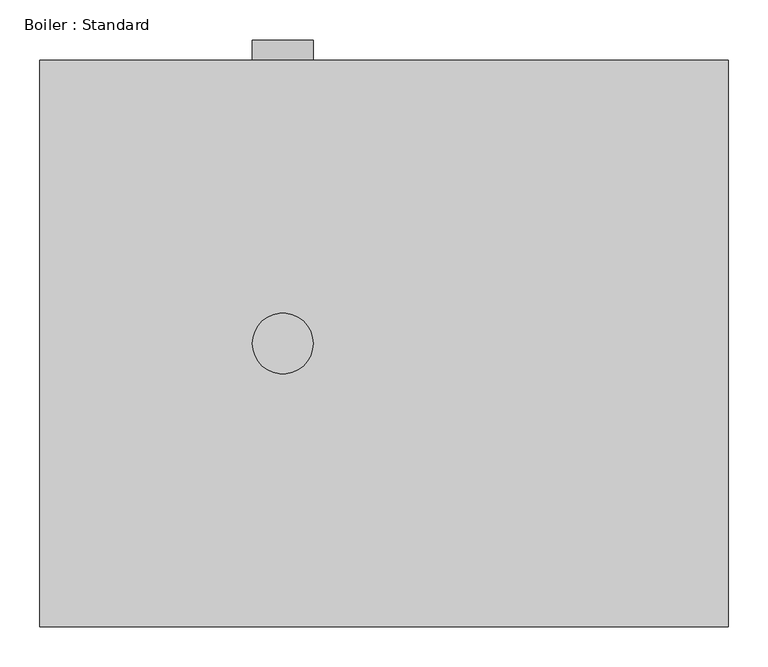
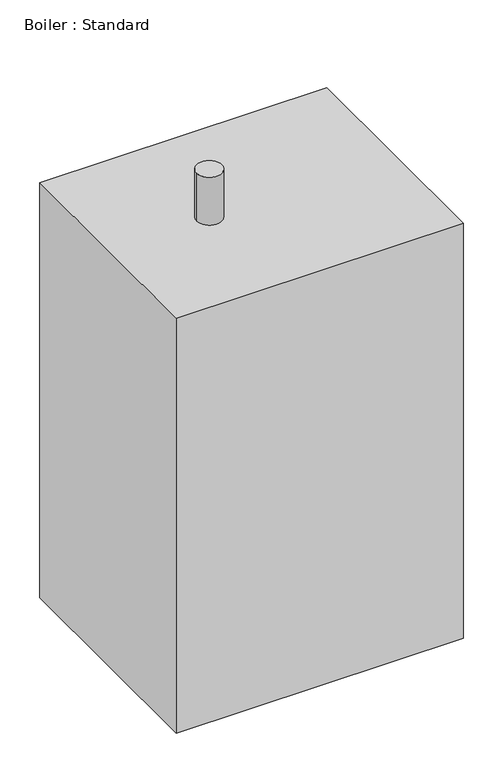
"""IFC4 building model written with IfcOpenShell, lengths in millimetres: proxy geometry, Boiler : Standard."""

from ifc_helpers import new_model, si_unit, point, frame, frame_2d, origin, origin_with_axes, place, context, project, spatial, polyline, circle_curve, trimmed, segment, composite_curve, outline, extrude, source, transform, mapped, element, save


def boiler_standard_3ade9070(model_context):
    return source(origin(), model_context, "Body", "SweptSolid", [
        extrude(outline(composite_curve([segment(trimmed(circle_curve(frame_2d((254.0, 304.8)), 38.1), [point((254.0, 342.9))], [point((254.0, 266.7))], False, "CARTESIAN"), True, "CONTINUOUS"), segment(trimmed(circle_curve(frame_2d((254.0, 304.8)), 38.1), [point((254.0, 266.7))], [point((254.0, 342.9))], False, "CARTESIAN"), True, "CONTINUOUS")], self_intersect=False)), frame((0.0, 711.2, 0.0), z_axis=(0.0, 1.0, 0.0), x_axis=(0.0, 0.0, 1.0)), (0.0, 0.0, 1.0), 25.4),
        extrude(outline(composite_curve([segment(trimmed(circle_curve(frame_2d((304.8, 355.6)), 38.1), [point((266.7, 355.6))], [point((342.9, 355.6))], False, "CARTESIAN"), True, "CONTINUOUS"), segment(trimmed(circle_curve(frame_2d((304.8, 355.6)), 38.1), [point((342.9, 355.6))], [point((266.7, 355.6))], False, "CARTESIAN"), True, "CONTINUOUS")], self_intersect=False)), frame((0.0, 0.0, 1320.8), z_axis=(0.0, 0.0, 1.0), x_axis=(1.0, 0.0, 0.0)), (0.0, 0.0, 1.0), 152.4),
        extrude(outline(polyline([(863.6, 0.0), (0.0, 0.0), (0.0, 711.2), (863.6, 711.2), (863.6, 0.0)])), origin_with_axes(), (0.0, 0.0, 1.0), 1320.8),
    ])


if __name__ == "__main__":
    model = new_model("IFC4")
    model_context = context("Model", 3, world=origin())
    ifc_project = project(units=[si_unit("LENGTHUNIT", "METRE", prefix="MILLI")], contexts=[model_context])
    site = spatial("IfcSite", under=ifc_project)
    building = spatial("IfcBuilding", under=site)
    placement = place(None, origin())
    boiler_standard_shape = boiler_standard_3ade9070(model_context)
    element("IfcBuildingElementProxy", 1, Name="Boiler : Standard", ObjectType="Boiler : Standard", at=placement, inside=building, context=model_context, shape_type="MappedRepresentation", body=[
        mapped(boiler_standard_shape, transform((0.0, 0.0, 0.0), x_axis=(1.0, 0.0, 0.0), y_axis=(0.0, 1.0, 0.0), z_axis=(0.0, 0.0, 1.0))),
    ])
    save(model, "model.ifc")

# Revit data of these elements
# Project information
#   Project Issue Date = "Issue Date"
#   Project Status = "Project Status"
#   Client Name = "Owner"
#   Project Address = "Enter address here"
#   Project Name = "Project Name"
#   Project Number = "Project Number"
# Type "Boiler : Standard"
#   Pressure Drop [instance default] = 1.70 psi
#   Max Flow = 230 GPM
#   Connector = 1 1/2"
#   Assembly Code = ""
